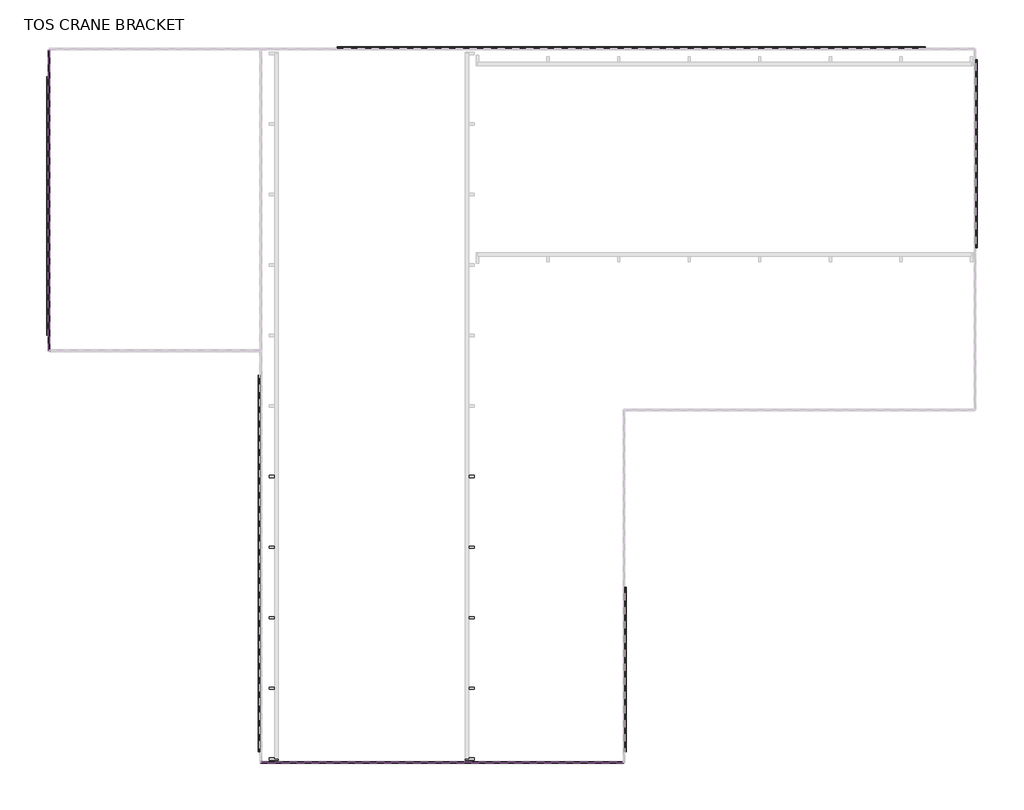
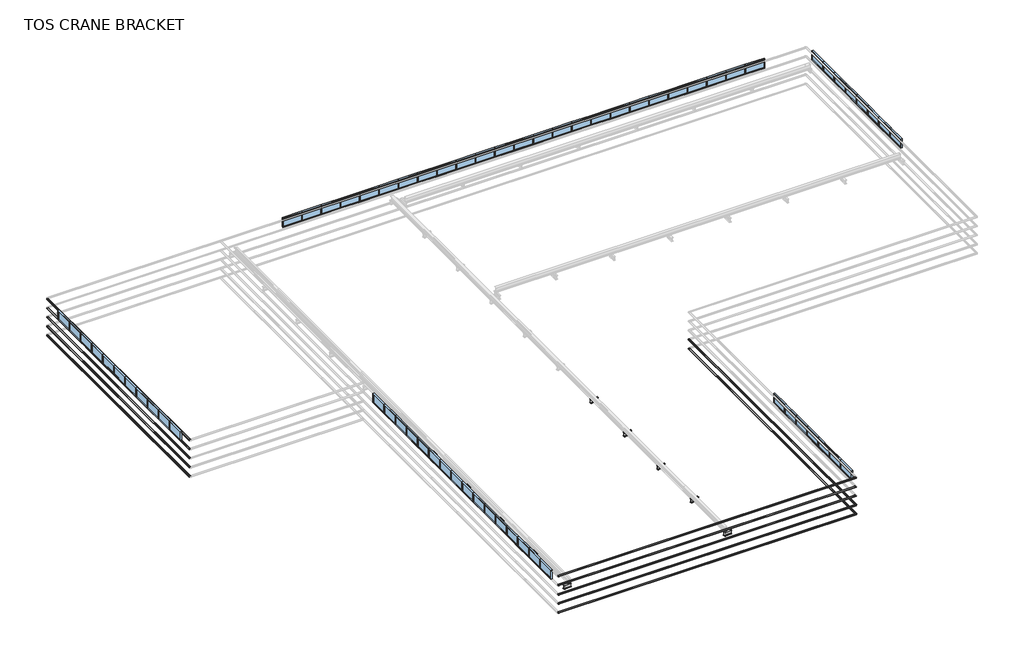
# One storey, part 1 of 3: 67 windows, 22 beams.
"""IFC4 building model written with IfcOpenShell, lengths in millimetres."""

import ifcopenshell
import ifcopenshell.guid

model = None  # the IFC model being written
_history = None  # IfcOwnerHistory: only IFC2X3 demands one
_inside = {}  # id of a spatial element -> (the spatial element, [elements in it])
_under = {}  # id of a project, library or spatial element -> (it, [spatial elements below it])
_declared = {}  # id of a project -> (the project, [libraries it declares])
_typed = {}  # id of a type object -> (the type object, [elements of that type])
_made_of = {}  # id of a material, layer set ... -> (it, [elements and type objects made of it])


def new_model(schema):
    """Start an empty IFC model of exactly this schema.

    Asked for "IFC4X3", IfcOpenShell would pick the latest addendum, in which some entities
    have other attributes; the version numbers below select the first issue.
    IFC2X3 requires an IfcOwnerHistory on every rooted entity: one is made here for all.
    """
    global model, _history
    if schema == "IFC4X3":
        model = ifcopenshell.file(schema_version=(4, 3, 0, 0))
    else:
        model = ifcopenshell.file(schema=schema)
    _inside.clear()
    _under.clear()
    _declared.clear()
    _typed.clear()
    _made_of.clear()
    _history = None
    if model.schema == "IFC2X3":
        org = make("IfcOrganization", Name="unknown")
        user = make(
            "IfcPersonAndOrganization",
            ThePerson=make("IfcPerson", FamilyName="unknown"),
            TheOrganization=org,
        )
        app = make(
            "IfcApplication",
            ApplicationDeveloper=org,
            Version="unknown",
            ApplicationFullName="unknown",
            ApplicationIdentifier="unknown",
        )
        _history = make(
            "IfcOwnerHistory",
            OwningUser=user,
            OwningApplication=app,
            ChangeAction="ADDED",
            CreationDate=0,
        )
    return model


def make(cls, **values):
    """One entity of the class cls with the attributes given. An attribute that is None is left unset."""
    return model.create_entity(
        cls, **{name: value for name, value in values.items() if value is not None}
    )


def rooted(cls, **values):
    """An entity with a GlobalId (a new one), such as an element, a storey or a relation."""
    return make(cls, GlobalId=ifcopenshell.guid.new(), OwnerHistory=_history, **values)


def si_unit(unit_type, name, prefix=None):
    """IfcSIUnit, for example si_unit("LENGTHUNIT", "METRE", prefix="MILLI")."""
    return make("IfcSIUnit", UnitType=unit_type, Prefix=prefix, Name=name)


def assignment(units):
    """IfcUnitAssignment: the units of a project."""
    return None if units is None else make("IfcUnitAssignment", Units=units)


def point(xyz):
    """IfcCartesianPoint."""
    return None if xyz is None else make("IfcCartesianPoint", Coordinates=xyz)


def direction(xyz):
    """IfcDirection."""
    return None if xyz is None else make("IfcDirection", DirectionRatios=xyz)


def frame(location, z_axis=None, x_axis=None):
    """IfcAxis2Placement3D, a coordinate frame: its origin and axes. An axis left out is left unset."""
    return make(
        "IfcAxis2Placement3D",
        Location=point(location),
        Axis=direction(z_axis),
        RefDirection=direction(x_axis),
    )


def frame_2d(location, x_axis=None):
    """IfcAxis2Placement2D, a coordinate frame in the plane: its origin and x axis."""
    return make(
        "IfcAxis2Placement2D", Location=point(location), RefDirection=direction(x_axis)
    )


def origin():
    """The frame at (0, 0, 0) with its axes left unset."""
    return frame((0.0, 0.0, 0.0))


def place(relative_to, where):
    """IfcLocalPlacement: puts the frame where relative to a parent placement (None: the world)."""
    return make(
        "IfcLocalPlacement", PlacementRelTo=relative_to, RelativePlacement=where
    )


def context(
    kind, dimensions, precision=None, world=None, true_north=None, identifier=None
):
    """IfcGeometricRepresentationContext, for example the 3D "Model" context."""
    return make(
        "IfcGeometricRepresentationContext",
        ContextIdentifier=identifier,
        ContextType=kind,
        CoordinateSpaceDimension=dimensions,
        Precision=precision,
        WorldCoordinateSystem=world,
        TrueNorth=true_north,
    )


def project(units=None, contexts=None):
    """IfcProject with its units and contexts."""
    return rooted(
        "IfcProject",
        Name="project",
        RepresentationContexts=contexts,
        UnitsInContext=assignment(units),
    )


def spatial(cls, under=None, at=None, **own):
    """A site, building, storey or space (cls), placed at a placement, below another one or the project."""
    s = rooted(cls, ObjectPlacement=at, **own)
    if under is not None:
        _under.setdefault(under.id(), (under, []))[1].append(s)
    return s


def polyline(points):
    """IfcPolyline through the points."""
    return make("IfcPolyline", Points=[point(p) for p in points])


def circle_curve(where, radius):
    """IfcCircle in the frame where."""
    return make("IfcCircle", Position=where, Radius=radius)


def trimmed(basis, trim1, trim2, sense, master):
    """IfcTrimmedCurve: the piece of a basis curve between two trims."""
    return make(
        "IfcTrimmedCurve",
        BasisCurve=basis,
        Trim1=trim1,
        Trim2=trim2,
        SenseAgreement=sense,
        MasterRepresentation=master,
    )


def segment(curve, same_sense, transition):
    """IfcCompositeCurveSegment."""
    return make(
        "IfcCompositeCurveSegment",
        Transition=transition,
        SameSense=same_sense,
        ParentCurve=curve,
    )


def composite_curve(segments, self_intersect=None):
    """IfcCompositeCurve: segments joined end to end."""
    return make("IfcCompositeCurve", Segments=segments, SelfIntersect=self_intersect)


def outline(outer, holes=None, kind="AREA"):
    """IfcArbitraryClosedProfileDef: a profile drawn as a closed curve; with holes, ...WithVoids."""
    if holes is None:
        return make("IfcArbitraryClosedProfileDef", ProfileType=kind, OuterCurve=outer)
    return make(
        "IfcArbitraryProfileDefWithVoids",
        ProfileType=kind,
        OuterCurve=outer,
        InnerCurves=holes,
    )


def extrude(swept, where, along, depth):
    """IfcExtrudedAreaSolid: the profile swept, set in the frame where, extruded along a direction by depth."""
    return make(
        "IfcExtrudedAreaSolid",
        SweptArea=swept,
        Position=where,
        ExtrudedDirection=direction(along),
        Depth=depth,
    )


def shape(context_of_items, identifier, shape_type, items):
    """IfcShapeRepresentation: the items that make up one representation, for example the "Body"."""
    return make(
        "IfcShapeRepresentation",
        ContextOfItems=context_of_items,
        RepresentationIdentifier=identifier,
        RepresentationType=shape_type,
        Items=items,
    )


def source(mapping_origin, context_of_items, identifier, shape_type, items):
    """IfcRepresentationMap: a shape defined once, which mapped items show again and again."""
    return make(
        "IfcRepresentationMap",
        MappingOrigin=mapping_origin,
        MappedRepresentation=shape(context_of_items, identifier, shape_type, items),
    )


def transform(
    local_origin,
    x_axis=None,
    y_axis=None,
    z_axis=None,
    scale=None,
    scale2=None,
    scale3=None,
    uniform=True,
):
    """IfcCartesianTransformationOperator3D, or its non-uniform kind. x_axis, y_axis, z_axis: its Axis1, 2, 3."""
    if uniform:
        return make(
            "IfcCartesianTransformationOperator3D",
            Axis1=direction(x_axis),
            Axis2=direction(y_axis),
            LocalOrigin=point(local_origin),
            Scale=scale,
            Axis3=direction(z_axis),
        )
    return make(
        "IfcCartesianTransformationOperator3DnonUniform",
        Axis1=direction(x_axis),
        Axis2=direction(y_axis),
        LocalOrigin=point(local_origin),
        Scale=scale,
        Axis3=direction(z_axis),
        Scale2=scale2,
        Scale3=scale3,
    )


def mapped(mapping_source, mapping_target):
    """IfcMappedItem: shows the shape of a source again, moved by a transform."""
    return make(
        "IfcMappedItem", MappingSource=mapping_source, MappingTarget=mapping_target
    )


def made_of(thing, what):
    """Note that an element or type object is made of a material, layer set ...; save() writes the relation."""
    if what is not None:
        _made_of.setdefault(what.id(), (what, []))[1].append(thing)
    return thing


def element(
    cls,
    number,
    at=None,
    inside=None,
    cuts=None,
    type_object=None,
    material=None,
    context=None,
    identifier="Body",
    shape_type=None,
    held_by="IfcProductDefinitionShape",
    body=None,
    shapes=None,
    **own,
):
    """One element of the class cls, such as IfcWall. Its Tag is "e" and its number.

    at: its placement. inside: the storey or other place that contains it. cuts: it is an
    opening in that element (IfcRelVoidsElement). A single representation is given by context,
    identifier, shape_type and body (its items); several are given by shapes. held_by: the class
    of the entity that holds the representations. save() writes the other relations.
    """
    e = rooted(cls, Tag="e%d" % number, ObjectPlacement=at, **own)
    if body is not None:
        shapes = [shape(context, identifier, shape_type, body)]
    if shapes is not None:
        e.Representation = make(held_by, Representations=shapes)
    if inside is not None:
        _inside.setdefault(inside.id(), (inside, []))[1].append(e)
    if cuts is not None:
        rooted(
            "IfcRelVoidsElement", RelatingBuildingElement=cuts, RelatedOpeningElement=e
        )
    if type_object is not None:
        _typed.setdefault(type_object.id(), (type_object, []))[1].append(e)
    return made_of(e, material)


def aggregate(whole, parts):
    """IfcRelAggregates: a whole, such as a stair, and the parts it consists of."""
    return rooted("IfcRelAggregates", RelatingObject=whole, RelatedObjects=parts)


def save(model, path):
    """Write the relations noted so far, then the file.

    IfcRelAggregates (storeys below a building ...), IfcRelContainedInSpatialStructure (elements
    in a storey), IfcRelDefinesByType, IfcRelAssociatesMaterial and IfcRelDeclares: one each for
    every whole, place, type object, material and project.
    """
    for whole, parts in _under.values():
        aggregate(whole, parts)
    for where, things in _inside.values():
        rooted(
            "IfcRelContainedInSpatialStructure",
            RelatedElements=things,
            RelatingStructure=where,
        )
    for kind, things in _typed.values():
        rooted("IfcRelDefinesByType", RelatedObjects=things, RelatingType=kind)
    for what, things in _made_of.values():
        rooted("IfcRelAssociatesMaterial", RelatedObjects=things, RelatingMaterial=what)
    for by, libraries in _declared.values():
        rooted("IfcRelDeclares", RelatingContext=by, RelatedDefinitions=libraries)
    model.write(path)


def beam_a081c7c9(model_context):
    return source(origin(), model_context, "Body", "SweptSolid", [
        extrude(outline(composite_curve([segment(polyline([(100.0, -187.0), (100.0, -200.0), (-100.0, -200.0), (-100.0, -187.0), (-20.0, -187.0)]), True, "CONTINUOUS"), segment(trimmed(circle_curve(frame_2d((-20.0, -171.0)), 16.0), [point((-20.0, -187.0))], [point((-4.0, -171.0))], True, "CARTESIAN"), True, "CONTINUOUS"), segment(polyline([(-4.0, -171.0), (-4.0, 171.0)]), True, "CONTINUOUS"), segment(trimmed(circle_curve(frame_2d((-20.0, 171.0)), 16.0), [point((-4.0, 171.0))], [point((-20.0, 187.0))], True, "CARTESIAN"), True, "CONTINUOUS"), segment(polyline([(-20.0, 187.0), (-100.0, 187.0), (-100.0, 200.0), (100.0, 200.0), (100.0, 187.0), (20.0, 187.0)]), True, "CONTINUOUS"), segment(trimmed(circle_curve(frame_2d((20.0, 171.0)), 16.0), [point((20.0, 187.0))], [point((4.0, 171.0))], True, "CARTESIAN"), True, "CONTINUOUS"), segment(polyline([(4.0, 171.0), (4.0, -171.0)]), True, "CONTINUOUS"), segment(trimmed(circle_curve(frame_2d((20.0, -171.0)), 16.0), [point((4.0, -171.0))], [point((20.0, -187.0))], True, "CARTESIAN"), True, "CONTINUOUS"), segment(polyline([(20.0, -187.0), (100.0, -187.0)]), True, "CONTINUOUS")], self_intersect=False)), frame((-236.0, 0.0, 0.0), z_axis=(1.0, 0.0, 0.0), x_axis=(0.0, 1.0, 0.0)), (0.0, 0.0, 1.0), 766.0),
    ])


def beam_d36fe593(model_context):
    return source(origin(), model_context, "Body", "SweptSolid", [
        extrude(outline(composite_curve([segment(polyline([(-100.0, -187.0), (-20.0, -187.0)]), True, "CONTINUOUS"), segment(trimmed(circle_curve(frame_2d((-20.0, -171.0)), 16.0), [point((-20.0, -187.0))], [point((-4.0, -171.0))], True, "CARTESIAN"), True, "CONTINUOUS"), segment(polyline([(-4.0, -171.0), (-4.0, 171.0)]), True, "CONTINUOUS"), segment(trimmed(circle_curve(frame_2d((-20.0, 171.0)), 16.0), [point((-4.0, 171.0))], [point((-20.0, 187.0))], True, "CARTESIAN"), True, "CONTINUOUS"), segment(polyline([(-20.0, 187.0), (-100.0, 187.0), (-100.0, 200.0), (100.0, 200.0), (100.0, 187.0), (20.0, 187.0)]), True, "CONTINUOUS"), segment(trimmed(circle_curve(frame_2d((20.0, 171.0)), 16.0), [point((20.0, 187.0))], [point((4.0, 171.0))], True, "CARTESIAN"), True, "CONTINUOUS"), segment(polyline([(4.0, 171.0), (4.0, -171.0)]), True, "CONTINUOUS"), segment(trimmed(circle_curve(frame_2d((20.0, -171.0)), 16.0), [point((4.0, -171.0))], [point((20.0, -187.0))], True, "CARTESIAN"), True, "CONTINUOUS"), segment(polyline([(20.0, -187.0), (100.0, -187.0), (100.0, -200.0), (-100.0, -200.0), (-100.0, -187.0)]), True, "CONTINUOUS")], self_intersect=False)), frame((-236.0, 0.0, 0.0), z_axis=(1.0, 0.0, 0.0), x_axis=(0.0, 1.0, 0.0)), (0.0, 0.0, 1.0), 766.0),
    ])


def steel_framing_lc_f9ca99c4(model_context):
    return source(origin(), model_context, "Body", "SweptSolid", [
        extrude(outline(composite_curve([segment(polyline([(18.6, 67.0), (18.6, -67.0)]), True, "CONTINUOUS"), segment(trimmed(circle_curve(frame_2d((10.6, -67.0)), 8.0), [point((18.6, -67.0))], [point((10.6, -75.0))], False, "CARTESIAN"), True, "CONTINUOUS"), segment(polyline([(10.6, -75.0), (-48.4, -75.0)]), True, "CONTINUOUS"), segment(trimmed(circle_curve(frame_2d((-48.4, -67.0)), 8.0), [point((-48.4, -75.0))], [point((-56.4, -67.0))], False, "CARTESIAN"), True, "CONTINUOUS"), segment(polyline([(-56.4, -67.0), (-56.4, -50.0), (-53.2, -50.0), (-53.2, -67.0)]), True, "CONTINUOUS"), segment(trimmed(circle_curve(frame_2d((-48.4, -67.0)), 4.8), [point((-53.2, -67.0))], [point((-48.4, -71.8))], True, "CARTESIAN"), True, "CONTINUOUS"), segment(polyline([(-48.4, -71.8), (10.6, -71.8)]), True, "CONTINUOUS"), segment(trimmed(circle_curve(frame_2d((10.6, -67.0)), 4.8), [point((10.6, -71.8))], [point((15.4, -67.0))], True, "CARTESIAN"), True, "CONTINUOUS"), segment(polyline([(15.4, -67.0), (15.4, 67.0)]), True, "CONTINUOUS"), segment(trimmed(circle_curve(frame_2d((10.6, 67.0)), 4.8), [point((15.4, 67.0))], [point((10.6, 71.8))], True, "CARTESIAN"), True, "CONTINUOUS"), segment(polyline([(10.6, 71.8), (-48.4, 71.8)]), True, "CONTINUOUS"), segment(trimmed(circle_curve(frame_2d((-48.4, 67.0)), 4.8), [point((-48.4, 71.8))], [point((-53.2, 67.0))], True, "CARTESIAN"), True, "CONTINUOUS"), segment(polyline([(-53.2, 67.0), (-53.2, 50.0), (-56.4, 50.0), (-56.4, 67.0)]), True, "CONTINUOUS"), segment(trimmed(circle_curve(frame_2d((-48.4, 67.0)), 8.0), [point((-56.4, 67.0))], [point((-48.4, 75.0))], False, "CARTESIAN"), True, "CONTINUOUS"), segment(polyline([(-48.4, 75.0), (10.6, 75.0)]), True, "CONTINUOUS"), segment(trimmed(circle_curve(frame_2d((10.6, 67.0)), 8.0), [point((10.6, 75.0))], [point((18.6, 67.0))], False, "CARTESIAN"), True, "CONTINUOUS")], self_intersect=False)), frame((-12797.0, 0.0, 0.0), z_axis=(1.0, 0.0, 0.0), x_axis=(0.0, 1.0, 0.0)), (0.0, 0.0, 1.0), 25581.0),
    ])


def steel_framing_lc_7a68255c(model_context):
    return source(origin(), model_context, "Body", "SweptSolid", [
        extrude(outline(composite_curve([segment(polyline([(18.6, 67.0), (18.6, -67.0)]), True, "CONTINUOUS"), segment(trimmed(circle_curve(frame_2d((10.6, -67.0)), 8.0), [point((18.6, -67.0))], [point((10.6, -75.0))], False, "CARTESIAN"), True, "CONTINUOUS"), segment(polyline([(10.6, -75.0), (-48.4, -75.0)]), True, "CONTINUOUS"), segment(trimmed(circle_curve(frame_2d((-48.4, -67.0)), 8.0), [point((-48.4, -75.0))], [point((-56.4, -67.0))], False, "CARTESIAN"), True, "CONTINUOUS"), segment(polyline([(-56.4, -67.0), (-56.4, -50.0), (-53.2, -50.0), (-53.2, -67.0)]), True, "CONTINUOUS"), segment(trimmed(circle_curve(frame_2d((-48.4, -67.0)), 4.8), [point((-53.2, -67.0))], [point((-48.4, -71.8))], True, "CARTESIAN"), True, "CONTINUOUS"), segment(polyline([(-48.4, -71.8), (10.6, -71.8)]), True, "CONTINUOUS"), segment(trimmed(circle_curve(frame_2d((10.6, -67.0)), 4.8), [point((10.6, -71.8))], [point((15.4, -67.0))], True, "CARTESIAN"), True, "CONTINUOUS"), segment(polyline([(15.4, -67.0), (15.4, 67.0)]), True, "CONTINUOUS"), segment(trimmed(circle_curve(frame_2d((10.6, 67.0)), 4.8), [point((15.4, 67.0))], [point((10.6, 71.8))], True, "CARTESIAN"), True, "CONTINUOUS"), segment(polyline([(10.6, 71.8), (-48.4, 71.8)]), True, "CONTINUOUS"), segment(trimmed(circle_curve(frame_2d((-48.4, 67.0)), 4.8), [point((-48.4, 71.8))], [point((-53.2, 67.0))], True, "CARTESIAN"), True, "CONTINUOUS"), segment(polyline([(-53.2, 67.0), (-53.2, 50.0), (-56.4, 50.0), (-56.4, 67.0)]), True, "CONTINUOUS"), segment(trimmed(circle_curve(frame_2d((-48.4, 67.0)), 8.0), [point((-56.4, 67.0))], [point((-48.4, 75.0))], False, "CARTESIAN"), True, "CONTINUOUS"), segment(polyline([(-48.4, 75.0), (10.6, 75.0)]), True, "CONTINUOUS"), segment(trimmed(circle_curve(frame_2d((10.6, 67.0)), 8.0), [point((10.6, 75.0))], [point((18.6, 67.0))], False, "CARTESIAN"), True, "CONTINUOUS")], self_intersect=False)), frame((-15450.0, 0.0, 0.0), z_axis=(1.0, 0.0, 0.0), x_axis=(0.0, 1.0, 0.0)), (0.0, 0.0, 1.0), 30900.0),
    ])


def fixed_window_a76b3388(model_context):
    return source(origin(), model_context, "Body", "SweptSolid", [
        extrude(outline(polyline([(-950.0, 3.0), (950.0, 3.0), (950.0, -3.0), (-950.0, -3.0), (-950.0, 3.0)])), frame((0.0, 0.0, 850.0), z_axis=(0.0, 0.0, 1.0), x_axis=(1.0, 0.0, 0.0)), (0.0, 0.0, 1.0), 900.0),
        extrude(outline(polyline([(1800.0, -1000.0), (800.0, -1000.0), (800.0, 1000.0), (1800.0, 1000.0), (1800.0, -1000.0)]), holes=[polyline([(1750.0, -950.0), (1750.0, 950.0), (850.0, 950.0), (850.0, -950.0), (1750.0, -950.0)])]), frame((0.0, -75.0, 0.0), z_axis=(0.0, 1.0, 0.0), x_axis=(0.0, 0.0, 1.0)), (0.0, 0.0, 1.0), 150.0),
    ])


model = new_model("IFC4")

# Units and contexts
model_context = context("Model", 3, world=origin())
ifc_project = project(units=[si_unit("LENGTHUNIT", "METRE", prefix="MILLI")], contexts=[model_context])

# Site, building, storey
site = spatial("IfcSite", under=ifc_project)
building = spatial("IfcBuilding", under=site)
storey = spatial("IfcBuildingStorey", under=building, Name="TOS CRANE BRACKET", Elevation=6699.9618634)

# Beams
placement = place(None, origin())
beam_shape = beam_a081c7c9(model_context)
element("IfcBeam", 1, ObjectType="Steel Framing_H_KS : H_SB_AR_S02_H-400x200x8x13_SCB1", at=placement, inside=storey, context=model_context, shape_type="MappedRepresentation", body=[
    mapped(beam_shape, transform((35470.0, -36000.0, 6499.9618634), x_axis=(-1.0, 0.0, 0.0), y_axis=(0.0, -1.0, 0.0), z_axis=(0.0, 0.0, 1.0))),
])
element("IfcBeam", 2, ObjectType="Steel Framing_H_KS : H_SB_AR_S02_H-400x200x8x13_SCB1", at=placement, inside=storey, context=model_context, shape_type="MappedRepresentation", body=[
    mapped(beam_shape, transform((35470.0, -42000.0, 6499.9618634), x_axis=(-1.0, 0.0, 0.0), y_axis=(0.0, -1.0, 0.0), z_axis=(0.0, 0.0, 1.0))),
])
element("IfcBeam", 3, ObjectType="Steel Framing_H_KS : H_SB_AR_S02_H-400x200x8x13_SCB1", at=placement, inside=storey, context=model_context, shape_type="MappedRepresentation", body=[
    mapped(beam_shape, transform((35470.0, -48000.0, 6499.9618634), x_axis=(-1.0, 0.0, 0.0), y_axis=(0.0, -1.0, 0.0), z_axis=(0.0, 0.0, 1.0))),
])
element("IfcBeam", 4, ObjectType="Steel Framing_H_KS : H_SB_AR_S02_H-400x200x8x13_SCB1", at=placement, inside=storey, context=model_context, shape_type="MappedRepresentation", body=[
    mapped(beam_shape, transform((35470.0, -54000.0, 6499.9618634), x_axis=(-1.0, 0.0, 0.0), y_axis=(0.0, -1.0, 0.0), z_axis=(0.0, 0.0, 1.0))),
])
element("IfcBeam", 5, ObjectType="Steel Framing_H_KS : H_SB_AR_S02_H-400x200x8x13_SCB1", at=placement, inside=storey, context=model_context, shape_type="MappedRepresentation", body=[
    mapped(beam_shape, transform((35470.0, -60000.0, 6499.9618634), x_axis=(-1.0, 0.0, 0.0), y_axis=(0.0, -1.0, 0.0), z_axis=(0.0, 0.0, 1.0))),
])
beam_2_shape = beam_d36fe593(model_context)
element("IfcBeam", 6, ObjectType="Steel Framing_H_KS : H_SB_AR_S02_H-400x200x8x13_SCB1", at=placement, inside=storey, context=model_context, shape_type="MappedRepresentation", body=[
    mapped(beam_2_shape, transform((18530.0, -36000.0, 6499.9618634), x_axis=(1.0, 0.0, 0.0), y_axis=(0.0, 1.0, 0.0), z_axis=(0.0, 0.0, 1.0))),
])
element("IfcBeam", 7, ObjectType="Steel Framing_H_KS : H_SB_AR_S02_H-400x200x8x13_SCB1", at=placement, inside=storey, context=model_context, shape_type="MappedRepresentation", body=[
    mapped(beam_2_shape, transform((18530.0, -42000.0, 6499.9618634), x_axis=(1.0, 0.0, 0.0), y_axis=(0.0, 1.0, 0.0), z_axis=(0.0, 0.0, 1.0))),
])
element("IfcBeam", 8, ObjectType="Steel Framing_H_KS : H_SB_AR_S02_H-400x200x8x13_SCB1", at=placement, inside=storey, context=model_context, shape_type="MappedRepresentation", body=[
    mapped(beam_2_shape, transform((18530.0, -48000.0, 6499.9618634), x_axis=(1.0, 0.0, 0.0), y_axis=(0.0, 1.0, 0.0), z_axis=(0.0, 0.0, 1.0))),
])
element("IfcBeam", 9, ObjectType="Steel Framing_H_KS : H_SB_AR_S02_H-400x200x8x13_SCB1", at=placement, inside=storey, context=model_context, shape_type="MappedRepresentation", body=[
    mapped(beam_2_shape, transform((18530.0, -54000.0, 6499.9618634), x_axis=(1.0, 0.0, 0.0), y_axis=(0.0, 1.0, 0.0), z_axis=(0.0, 0.0, 1.0))),
])
element("IfcBeam", 10, ObjectType="Steel Framing_H_KS : H_SB_AR_S02_H-400x200x8x13_SCB1", at=placement, inside=storey, context=model_context, shape_type="MappedRepresentation", body=[
    mapped(beam_2_shape, transform((18530.0, -60000.0, 6499.9618634), x_axis=(1.0, 0.0, 0.0), y_axis=(0.0, 1.0, 0.0), z_axis=(0.0, 0.0, 1.0))),
])
element("IfcBeam", 11, ObjectType="Steel Framing_LC : H_SB_AR_S00_LC-150x75x25x3.2", at=placement, inside=storey, context=model_context, shape_type="SweptSolid", body=[
    extrude(outline(composite_curve([segment(polyline([(4168.5618634, 48517.0), (4168.5618634, 48383.0)]), True, "CONTINUOUS"), segment(trimmed(circle_curve(frame_2d((4160.5618634, 48383.0)), 8.0), [point((4168.5618634, 48383.0))], [point((4160.5618634, 48375.0))], False, "CARTESIAN"), True, "CONTINUOUS"), segment(polyline([(4160.5618634, 48375.0), (4101.5618634, 48375.0)]), True, "CONTINUOUS"), segment(trimmed(circle_curve(frame_2d((4101.5618634, 48383.0)), 8.0), [point((4101.5618634, 48375.0))], [point((4093.5618634, 48383.0))], False, "CARTESIAN"), True, "CONTINUOUS"), segment(polyline([(4093.5618634, 48383.0), (4093.5618634, 48400.0), (4096.7618634, 48400.0), (4096.7618634, 48383.0)]), True, "CONTINUOUS"), segment(trimmed(circle_curve(frame_2d((4101.5618634, 48383.0)), 4.8), [point((4096.7618634, 48383.0))], [point((4101.5618634, 48378.2))], True, "CARTESIAN"), True, "CONTINUOUS"), segment(polyline([(4101.5618634, 48378.2), (4160.5618634, 48378.2)]), True, "CONTINUOUS"), segment(trimmed(circle_curve(frame_2d((4160.5618634, 48383.0)), 4.8), [point((4160.5618634, 48378.2))], [point((4165.3618634, 48383.0))], True, "CARTESIAN"), True, "CONTINUOUS"), segment(polyline([(4165.3618634, 48383.0), (4165.3618634, 48517.0)]), True, "CONTINUOUS"), segment(trimmed(circle_curve(frame_2d((4160.5618634, 48517.0)), 4.8), [point((4165.3618634, 48517.0))], [point((4160.5618634, 48521.8))], True, "CARTESIAN"), True, "CONTINUOUS"), segment(polyline([(4160.5618634, 48521.8), (4101.5618634, 48521.8)]), True, "CONTINUOUS"), segment(trimmed(circle_curve(frame_2d((4101.5618634, 48517.0)), 4.8), [point((4101.5618634, 48521.8))], [point((4096.7618634, 48517.0))], True, "CARTESIAN"), True, "CONTINUOUS"), segment(polyline([(4096.7618634, 48517.0), (4096.7618634, 48500.0), (4093.5618634, 48500.0), (4093.5618634, 48517.0)]), True, "CONTINUOUS"), segment(trimmed(circle_curve(frame_2d((4101.5618634, 48517.0)), 8.0), [point((4093.5618634, 48517.0))], [point((4101.5618634, 48525.0))], False, "CARTESIAN"), True, "CONTINUOUS"), segment(polyline([(4101.5618634, 48525.0), (4160.5618634, 48525.0)]), True, "CONTINUOUS"), segment(trimmed(circle_curve(frame_2d((4160.5618634, 48517.0)), 8.0), [point((4160.5618634, 48525.0))], [point((4168.5618634, 48517.0))], False, "CARTESIAN"), True, "CONTINUOUS")], self_intersect=False)), frame((0.0, -60300.0, 0.0), z_axis=(0.0, 1.0, 0.0), x_axis=(0.0, 0.0, 1.0)), (0.0, 0.0, 1.0), 29975.0),
])
element("IfcBeam", 12, ObjectType="Steel Framing_LC : H_SB_AR_S00_LC-150x75x25x3.2", at=placement, inside=storey, context=model_context, shape_type="SweptSolid", body=[
    extrude(outline(composite_curve([segment(polyline([(5168.5618634, 48517.0), (5168.5618634, 48383.0)]), True, "CONTINUOUS"), segment(trimmed(circle_curve(frame_2d((5160.5618634, 48383.0)), 8.0), [point((5168.5618634, 48383.0))], [point((5160.5618634, 48375.0))], False, "CARTESIAN"), True, "CONTINUOUS"), segment(polyline([(5160.5618634, 48375.0), (5101.5618634, 48375.0)]), True, "CONTINUOUS"), segment(trimmed(circle_curve(frame_2d((5101.5618634, 48383.0)), 8.0), [point((5101.5618634, 48375.0))], [point((5093.5618634, 48383.0))], False, "CARTESIAN"), True, "CONTINUOUS"), segment(polyline([(5093.5618634, 48383.0), (5093.5618634, 48400.0), (5096.7618634, 48400.0), (5096.7618634, 48383.0)]), True, "CONTINUOUS"), segment(trimmed(circle_curve(frame_2d((5101.5618634, 48383.0)), 4.8), [point((5096.7618634, 48383.0))], [point((5101.5618634, 48378.2))], True, "CARTESIAN"), True, "CONTINUOUS"), segment(polyline([(5101.5618634, 48378.2), (5160.5618634, 48378.2)]), True, "CONTINUOUS"), segment(trimmed(circle_curve(frame_2d((5160.5618634, 48383.0)), 4.8), [point((5160.5618634, 48378.2))], [point((5165.3618634, 48383.0))], True, "CARTESIAN"), True, "CONTINUOUS"), segment(polyline([(5165.3618634, 48383.0), (5165.3618634, 48517.0)]), True, "CONTINUOUS"), segment(trimmed(circle_curve(frame_2d((5160.5618634, 48517.0)), 4.8), [point((5165.3618634, 48517.0))], [point((5160.5618634, 48521.8))], True, "CARTESIAN"), True, "CONTINUOUS"), segment(polyline([(5160.5618634, 48521.8), (5101.5618634, 48521.8)]), True, "CONTINUOUS"), segment(trimmed(circle_curve(frame_2d((5101.5618634, 48517.0)), 4.8), [point((5101.5618634, 48521.8))], [point((5096.7618634, 48517.0))], True, "CARTESIAN"), True, "CONTINUOUS"), segment(polyline([(5096.7618634, 48517.0), (5096.7618634, 48500.0), (5093.5618634, 48500.0), (5093.5618634, 48517.0)]), True, "CONTINUOUS"), segment(trimmed(circle_curve(frame_2d((5101.5618634, 48517.0)), 8.0), [point((5093.5618634, 48517.0))], [point((5101.5618634, 48525.0))], False, "CARTESIAN"), True, "CONTINUOUS"), segment(polyline([(5101.5618634, 48525.0), (5160.5618634, 48525.0)]), True, "CONTINUOUS"), segment(trimmed(circle_curve(frame_2d((5160.5618634, 48517.0)), 8.0), [point((5160.5618634, 48525.0))], [point((5168.5618634, 48517.0))], False, "CARTESIAN"), True, "CONTINUOUS")], self_intersect=False)), frame((0.0, -60300.0, 0.0), z_axis=(0.0, 1.0, 0.0), x_axis=(0.0, 0.0, 1.0)), (0.0, 0.0, 1.0), 29975.0),
])
steel_framing_lc_shape = steel_framing_lc_f9ca99c4(model_context)
element("IfcBeam", 13, ObjectType="Steel Framing_LC : H_SB_AR_S00_LC-150x75x25x3.2", at=placement, inside=storey, context=model_context, shape_type="MappedRepresentation", body=[
    mapped(steel_framing_lc_shape, transform((-450.0, -12503.0, 4149.9618634), x_axis=(0.0, 1.0, 0.0), y_axis=(0.0, 0.0, 1.0), z_axis=(1.0, 0.0, 0.0))),
])
element("IfcBeam", 14, ObjectType="Steel Framing_LC : H_SB_AR_S00_LC-150x75x25x3.2", at=placement, inside=storey, context=model_context, shape_type="MappedRepresentation", body=[
    mapped(steel_framing_lc_shape, transform((-450.0, -12503.0, 5149.9618634), x_axis=(0.0, 1.0, 0.0), y_axis=(0.0, 0.0, 1.0), z_axis=(1.0, 0.0, 0.0))),
])
element("IfcBeam", 15, ObjectType="Steel Framing_LC : H_SB_AR_S00_LC-150x75x25x3.2", at=placement, inside=storey, context=model_context, shape_type="MappedRepresentation", body=[
    mapped(steel_framing_lc_shape, transform((-450.0, -12503.0, 6149.9618634), x_axis=(0.0, 1.0, 0.0), y_axis=(0.0, 0.0, 1.0), z_axis=(1.0, 0.0, 0.0))),
])
element("IfcBeam", 16, ObjectType="Steel Framing_LC : H_SB_AR_S00_LC-150x75x25x3.2", at=placement, inside=storey, context=model_context, shape_type="MappedRepresentation", body=[
    mapped(steel_framing_lc_shape, transform((-450.0, -12503.0, 7149.9618634), x_axis=(0.0, 1.0, 0.0), y_axis=(0.0, 0.0, 1.0), z_axis=(1.0, 0.0, 0.0))),
])
element("IfcBeam", 17, ObjectType="Steel Framing_LC : H_SB_AR_S00_LC-150x75x25x3.2", at=placement, inside=storey, context=model_context, shape_type="MappedRepresentation", body=[
    mapped(steel_framing_lc_shape, transform((-450.0, -12503.0, 8149.9618634), x_axis=(0.0, 1.0, 0.0), y_axis=(0.0, 0.0, 1.0), z_axis=(1.0, 0.0, 0.0))),
])
steel_framing_lc_2_shape = steel_framing_lc_7a68255c(model_context)
element("IfcBeam", 18, ObjectType="Steel Framing_LC : H_SB_AR_S00_LC-150x75x25x3.2", at=placement, inside=storey, context=model_context, shape_type="MappedRepresentation", body=[
    mapped(steel_framing_lc_2_shape, transform((33000.0, -60300.0, 4149.9618634), x_axis=(1.0, 0.0, 0.0), y_axis=(0.0, 0.0, 1.0), z_axis=(0.0, -1.0, 0.0))),
])
element("IfcBeam", 19, ObjectType="Steel Framing_LC : H_SB_AR_S00_LC-150x75x25x3.2", at=placement, inside=storey, context=model_context, shape_type="MappedRepresentation", body=[
    mapped(steel_framing_lc_2_shape, transform((33000.0, -60300.0, 5149.9618634), x_axis=(1.0, 0.0, 0.0), y_axis=(0.0, 0.0, 1.0), z_axis=(0.0, -1.0, 0.0))),
])
element("IfcBeam", 20, ObjectType="Steel Framing_LC : H_SB_AR_S00_LC-150x75x25x3.2", at=placement, inside=storey, context=model_context, shape_type="MappedRepresentation", body=[
    mapped(steel_framing_lc_2_shape, transform((33000.0, -60300.0, 6149.9618634), x_axis=(1.0, 0.0, 0.0), y_axis=(0.0, 0.0, 1.0), z_axis=(0.0, -1.0, 0.0))),
])
element("IfcBeam", 21, ObjectType="Steel Framing_LC : H_SB_AR_S00_LC-150x75x25x3.2", at=placement, inside=storey, context=model_context, shape_type="MappedRepresentation", body=[
    mapped(steel_framing_lc_2_shape, transform((33000.0, -60300.0, 7149.9618634), x_axis=(1.0, 0.0, 0.0), y_axis=(0.0, 0.0, 1.0), z_axis=(0.0, -1.0, 0.0))),
])
element("IfcBeam", 22, ObjectType="Steel Framing_LC : H_SB_AR_S00_LC-150x75x25x3.2", at=placement, inside=storey, context=model_context, shape_type="MappedRepresentation", body=[
    mapped(steel_framing_lc_2_shape, transform((33000.0, -60300.0, 8149.9618634), x_axis=(1.0, 0.0, 0.0), y_axis=(0.0, 0.0, 1.0), z_axis=(0.0, -1.0, 0.0))),
])

# Windows
fixed_window_shape = fixed_window_a76b3388(model_context)
element("IfcWindow", 23, ObjectType="Fixed Window : H_WD_AR_B11_Fix_Steel Window_SG_W2000xH1000", at=placement, inside=storey, context=model_context, shape_type="MappedRepresentation", body=[
    mapped(fixed_window_shape, transform((-585.0, -22975.0, 6499.9618634), x_axis=(0.0, 1.0, 0.0), y_axis=(-1.0, 0.0, 0.0), z_axis=(0.0, 0.0, 1.0))),
])
element("IfcWindow", 24, ObjectType="Fixed Window : H_WD_AR_B11_Fix_Steel Window_SG_W2000xH1000", at=placement, inside=storey, context=model_context, shape_type="MappedRepresentation", body=[
    mapped(fixed_window_shape, transform((-585.0, -20975.0, 6499.9618634), x_axis=(0.0, -1.0, 0.0), y_axis=(1.0, 0.0, 0.0), z_axis=(0.0, 0.0, 1.0))),
])
element("IfcWindow", 25, ObjectType="Fixed Window : H_WD_AR_B11_Fix_Steel Window_SG_W2000xH1000", at=placement, inside=storey, context=model_context, shape_type="MappedRepresentation", body=[
    mapped(fixed_window_shape, transform((-585.0, -18975.0, 6499.9618634), x_axis=(0.0, -1.0, 0.0), y_axis=(1.0, 0.0, 0.0), z_axis=(0.0, 0.0, 1.0))),
])
element("IfcWindow", 26, ObjectType="Fixed Window : H_WD_AR_B11_Fix_Steel Window_SG_W2000xH1000", at=placement, inside=storey, context=model_context, shape_type="MappedRepresentation", body=[
    mapped(fixed_window_shape, transform((-585.0, -16975.0, 6499.9618634), x_axis=(0.0, -1.0, 0.0), y_axis=(1.0, 0.0, 0.0), z_axis=(0.0, 0.0, 1.0))),
])
element("IfcWindow", 27, ObjectType="Fixed Window : H_WD_AR_B11_Fix_Steel Window_SG_W2000xH1000", at=placement, inside=storey, context=model_context, shape_type="MappedRepresentation", body=[
    mapped(fixed_window_shape, transform((-585.0, -14975.0, 6499.9618634), x_axis=(0.0, -1.0, 0.0), y_axis=(1.0, 0.0, 0.0), z_axis=(0.0, 0.0, 1.0))),
])
element("IfcWindow", 28, ObjectType="Fixed Window : H_WD_AR_B11_Fix_Steel Window_SG_W2000xH1000", at=placement, inside=storey, context=model_context, shape_type="MappedRepresentation", body=[
    mapped(fixed_window_shape, transform((-585.0, -12975.0, 6499.9618634), x_axis=(0.0, -1.0, 0.0), y_axis=(1.0, 0.0, 0.0), z_axis=(0.0, 0.0, 1.0))),
])
element("IfcWindow", 29, ObjectType="Fixed Window : H_WD_AR_B11_Fix_Steel Window_SG_W2000xH1000", at=placement, inside=storey, context=model_context, shape_type="MappedRepresentation", body=[
    mapped(fixed_window_shape, transform((-585.0, -10975.0, 6499.9618634), x_axis=(0.0, -1.0, 0.0), y_axis=(1.0, 0.0, 0.0), z_axis=(0.0, 0.0, 1.0))),
])
element("IfcWindow", 30, ObjectType="Fixed Window : H_WD_AR_B11_Fix_Steel Window_SG_W2000xH1000", at=placement, inside=storey, context=model_context, shape_type="MappedRepresentation", body=[
    mapped(fixed_window_shape, transform((-585.0, -8975.0, 6499.9618634), x_axis=(0.0, -1.0, 0.0), y_axis=(1.0, 0.0, 0.0), z_axis=(0.0, 0.0, 1.0))),
])
element("IfcWindow", 31, ObjectType="Fixed Window : H_WD_AR_B11_Fix_Steel Window_SG_W2000xH1000", at=placement, inside=storey, context=model_context, shape_type="MappedRepresentation", body=[
    mapped(fixed_window_shape, transform((-585.0, -6975.0, 6499.9618634), x_axis=(0.0, -1.0, 0.0), y_axis=(1.0, 0.0, 0.0), z_axis=(0.0, 0.0, 1.0))),
])
element("IfcWindow", 32, ObjectType="Fixed Window : H_WD_AR_B11_Fix_Steel Window_SG_W2000xH1000", at=placement, inside=storey, context=model_context, shape_type="MappedRepresentation", body=[
    mapped(fixed_window_shape, transform((-585.0, -4975.0, 6499.9618634), x_axis=(0.0, -1.0, 0.0), y_axis=(1.0, 0.0, 0.0), z_axis=(0.0, 0.0, 1.0))),
])
element("IfcWindow", 33, ObjectType="Fixed Window : H_WD_AR_B11_Fix_Steel Window_SG_W2000xH1000", at=placement, inside=storey, context=model_context, shape_type="MappedRepresentation", body=[
    mapped(fixed_window_shape, transform((-585.0, -2975.0, 6499.9618634), x_axis=(0.0, -1.0, 0.0), y_axis=(1.0, 0.0, 0.0), z_axis=(0.0, 0.0, 1.0))),
])
element("IfcWindow", 34, ObjectType="Fixed Window : H_WD_AR_B11_Fix_Steel Window_SG_W2000xH1000", at=placement, inside=storey, context=model_context, shape_type="MappedRepresentation", body=[
    mapped(fixed_window_shape, transform((25075.0, 504.0, 6499.9618634), x_axis=(1.0, 0.0, 0.0), y_axis=(0.0, 1.0, 0.0), z_axis=(0.0, 0.0, 1.0))),
])
element("IfcWindow", 35, ObjectType="Fixed Window : H_WD_AR_B11_Fix_Steel Window_SG_W2000xH1000", at=placement, inside=storey, context=model_context, shape_type="MappedRepresentation", body=[
    mapped(fixed_window_shape, transform((27075.0, 504.0, 6499.9618634), x_axis=(1.0, 0.0, 0.0), y_axis=(0.0, 1.0, 0.0), z_axis=(0.0, 0.0, 1.0))),
])
element("IfcWindow", 36, ObjectType="Fixed Window : H_WD_AR_B11_Fix_Steel Window_SG_W2000xH1000", at=placement, inside=storey, context=model_context, shape_type="MappedRepresentation", body=[
    mapped(fixed_window_shape, transform((29075.0, 504.0, 6499.9618634), x_axis=(1.0, 0.0, 0.0), y_axis=(0.0, 1.0, 0.0), z_axis=(0.0, 0.0, 1.0))),
])
element("IfcWindow", 37, ObjectType="Fixed Window : H_WD_AR_B11_Fix_Steel Window_SG_W2000xH1000", at=placement, inside=storey, context=model_context, shape_type="MappedRepresentation", body=[
    mapped(fixed_window_shape, transform((31075.0, 504.0, 6499.9618634), x_axis=(-1.0, 0.0, 0.0), y_axis=(0.0, -1.0, 0.0), z_axis=(0.0, 0.0, 1.0))),
])
element("IfcWindow", 38, ObjectType="Fixed Window : H_WD_AR_B11_Fix_Steel Window_SG_W2000xH1000", at=placement, inside=storey, context=model_context, shape_type="MappedRepresentation", body=[
    mapped(fixed_window_shape, transform((33075.0, 504.0, 6499.9618634), x_axis=(1.0, 0.0, 0.0), y_axis=(0.0, 1.0, 0.0), z_axis=(0.0, 0.0, 1.0))),
])
element("IfcWindow", 39, ObjectType="Fixed Window : H_WD_AR_B11_Fix_Steel Window_SG_W2000xH1000", at=placement, inside=storey, context=model_context, shape_type="MappedRepresentation", body=[
    mapped(fixed_window_shape, transform((35075.0, 504.0, 6499.9618634), x_axis=(1.0, 0.0, 0.0), y_axis=(0.0, 1.0, 0.0), z_axis=(0.0, 0.0, 1.0))),
])
element("IfcWindow", 40, ObjectType="Fixed Window : H_WD_AR_B11_Fix_Steel Window_SG_W2000xH1000", at=placement, inside=storey, context=model_context, shape_type="MappedRepresentation", body=[
    mapped(fixed_window_shape, transform((37075.0, 504.0, 6499.9618634), x_axis=(1.0, 0.0, 0.0), y_axis=(0.0, 1.0, 0.0), z_axis=(0.0, 0.0, 1.0))),
])
element("IfcWindow", 41, ObjectType="Fixed Window : H_WD_AR_B11_Fix_Steel Window_SG_W2000xH1000", at=placement, inside=storey, context=model_context, shape_type="MappedRepresentation", body=[
    mapped(fixed_window_shape, transform((39075.0, 504.0, 6499.9618634), x_axis=(1.0, 0.0, 0.0), y_axis=(0.0, 1.0, 0.0), z_axis=(0.0, 0.0, 1.0))),
])
element("IfcWindow", 42, ObjectType="Fixed Window : H_WD_AR_B11_Fix_Steel Window_SG_W2000xH1000", at=placement, inside=storey, context=model_context, shape_type="MappedRepresentation", body=[
    mapped(fixed_window_shape, transform((41075.0, 504.0, 6499.9618634), x_axis=(1.0, 0.0, 0.0), y_axis=(0.0, 1.0, 0.0), z_axis=(0.0, 0.0, 1.0))),
])
element("IfcWindow", 43, ObjectType="Fixed Window : H_WD_AR_B11_Fix_Steel Window_SG_W2000xH1000", at=placement, inside=storey, context=model_context, shape_type="MappedRepresentation", body=[
    mapped(fixed_window_shape, transform((43075.0, 504.0, 6499.9618634), x_axis=(-1.0, 0.0, 0.0), y_axis=(0.0, -1.0, 0.0), z_axis=(0.0, 0.0, 1.0))),
])
element("IfcWindow", 44, ObjectType="Fixed Window : H_WD_AR_B11_Fix_Steel Window_SG_W2000xH1000", at=placement, inside=storey, context=model_context, shape_type="MappedRepresentation", body=[
    mapped(fixed_window_shape, transform((45075.0, 504.0, 6499.9618634), x_axis=(1.0, 0.0, 0.0), y_axis=(0.0, 1.0, 0.0), z_axis=(0.0, 0.0, 1.0))),
])
element("IfcWindow", 45, ObjectType="Fixed Window : H_WD_AR_B11_Fix_Steel Window_SG_W2000xH1000", at=placement, inside=storey, context=model_context, shape_type="MappedRepresentation", body=[
    mapped(fixed_window_shape, transform((47075.0, 504.0, 6499.9618634), x_axis=(1.0, 0.0, 0.0), y_axis=(0.0, 1.0, 0.0), z_axis=(0.0, 0.0, 1.0))),
])
element("IfcWindow", 46, ObjectType="Fixed Window : H_WD_AR_B11_Fix_Steel Window_SG_W2000xH1000", at=placement, inside=storey, context=model_context, shape_type="MappedRepresentation", body=[
    mapped(fixed_window_shape, transform((49075.0, 504.0, 6499.9618634), x_axis=(1.0, 0.0, 0.0), y_axis=(0.0, 1.0, 0.0), z_axis=(0.0, 0.0, 1.0))),
])
element("IfcWindow", 47, ObjectType="Fixed Window : H_WD_AR_B11_Fix_Steel Window_SG_W2000xH1000", at=placement, inside=storey, context=model_context, shape_type="MappedRepresentation", body=[
    mapped(fixed_window_shape, transform((51075.0, 504.0, 6499.9618634), x_axis=(1.0, 0.0, 0.0), y_axis=(0.0, 1.0, 0.0), z_axis=(0.0, 0.0, 1.0))),
])
element("IfcWindow", 48, ObjectType="Fixed Window : H_WD_AR_B11_Fix_Steel Window_SG_W2000xH1000", at=placement, inside=storey, context=model_context, shape_type="MappedRepresentation", body=[
    mapped(fixed_window_shape, transform((53075.0, 504.0, 6499.9618634), x_axis=(1.0, 0.0, 0.0), y_axis=(0.0, 1.0, 0.0), z_axis=(0.0, 0.0, 1.0))),
])
element("IfcWindow", 49, ObjectType="Fixed Window : H_WD_AR_B11_Fix_Steel Window_SG_W2000xH1000", at=placement, inside=storey, context=model_context, shape_type="MappedRepresentation", body=[
    mapped(fixed_window_shape, transform((55075.0, 504.0, 6499.9618634), x_axis=(1.0, 0.0, 0.0), y_axis=(0.0, 1.0, 0.0), z_axis=(0.0, 0.0, 1.0))),
])
element("IfcWindow", 50, ObjectType="Fixed Window : H_WD_AR_B11_Fix_Steel Window_SG_W2000xH1000", at=placement, inside=storey, context=model_context, shape_type="MappedRepresentation", body=[
    mapped(fixed_window_shape, transform((57075.0, 504.0, 6499.9618634), x_axis=(1.0, 0.0, 0.0), y_axis=(0.0, 1.0, 0.0), z_axis=(0.0, 0.0, 1.0))),
])
element("IfcWindow", 51, ObjectType="Fixed Window : H_WD_AR_B11_Fix_Steel Window_SG_W2000xH1000", at=placement, inside=storey, context=model_context, shape_type="MappedRepresentation", body=[
    mapped(fixed_window_shape, transform((59075.0, 504.0, 6499.9618634), x_axis=(1.0, 0.0, 0.0), y_axis=(0.0, 1.0, 0.0), z_axis=(0.0, 0.0, 1.0))),
])
element("IfcWindow", 52, ObjectType="Fixed Window : H_WD_AR_B11_Fix_Steel Window_SG_W2000xH1000", at=placement, inside=storey, context=model_context, shape_type="MappedRepresentation", body=[
    mapped(fixed_window_shape, transform((61075.0, 504.0, 6499.9618634), x_axis=(1.0, 0.0, 0.0), y_axis=(0.0, 1.0, 0.0), z_axis=(0.0, 0.0, 1.0))),
])
element("IfcWindow", 53, ObjectType="Fixed Window : H_WD_AR_B11_Fix_Steel Window_SG_W2000xH1000", at=placement, inside=storey, context=model_context, shape_type="MappedRepresentation", body=[
    mapped(fixed_window_shape, transform((63075.0, 504.0, 6499.9618634), x_axis=(1.0, 0.0, 0.0), y_axis=(0.0, 1.0, 0.0), z_axis=(0.0, 0.0, 1.0))),
])
element("IfcWindow", 54, ObjectType="Fixed Window : H_WD_AR_B11_Fix_Steel Window_SG_W2000xH1000", at=placement, inside=storey, context=model_context, shape_type="MappedRepresentation", body=[
    mapped(fixed_window_shape, transform((65075.0, 504.0, 6499.9618634), x_axis=(1.0, 0.0, 0.0), y_axis=(0.0, 1.0, 0.0), z_axis=(0.0, 0.0, 1.0))),
])
element("IfcWindow", 55, ObjectType="Fixed Window : H_WD_AR_B11_Fix_Steel Window_SG_W2000xH1000", at=placement, inside=storey, context=model_context, shape_type="MappedRepresentation", body=[
    mapped(fixed_window_shape, transform((67075.0, 504.0, 6499.9618634), x_axis=(1.0, 0.0, 0.0), y_axis=(0.0, 1.0, 0.0), z_axis=(0.0, 0.0, 1.0))),
])
element("IfcWindow", 56, ObjectType="Fixed Window : H_WD_AR_B11_Fix_Steel Window_SG_W2000xH1000", at=placement, inside=storey, context=model_context, shape_type="MappedRepresentation", body=[
    mapped(fixed_window_shape, transform((69075.0, 504.0, 6499.9618634), x_axis=(1.0, 0.0, 0.0), y_axis=(0.0, 1.0, 0.0), z_axis=(0.0, 0.0, 1.0))),
])
element("IfcWindow", 57, ObjectType="Fixed Window : H_WD_AR_B11_Fix_Steel Window_SG_W2000xH1000", at=placement, inside=storey, context=model_context, shape_type="MappedRepresentation", body=[
    mapped(fixed_window_shape, transform((71075.0, 504.0, 6499.9618634), x_axis=(1.0, 0.0, 0.0), y_axis=(0.0, 1.0, 0.0), z_axis=(0.0, 0.0, 1.0))),
])
element("IfcWindow", 58, ObjectType="Fixed Window : H_WD_AR_B11_Fix_Steel Window_SG_W2000xH1000", at=placement, inside=storey, context=model_context, shape_type="MappedRepresentation", body=[
    mapped(fixed_window_shape, transform((73075.0, 504.0, 6499.9618634), x_axis=(1.0, 0.0, 0.0), y_axis=(0.0, 1.0, 0.0), z_axis=(0.0, 0.0, 1.0))),
])
element("IfcWindow", 59, ObjectType="Fixed Window : H_WD_AR_B11_Fix_Steel Window_SG_W2000xH1000", at=placement, inside=storey, context=model_context, shape_type="MappedRepresentation", body=[
    mapped(fixed_window_shape, transform((78435.0, -1556.0, 6499.9618634), x_axis=(0.0, -1.0, 0.0), y_axis=(1.0, 0.0, 0.0), z_axis=(0.0, 0.0, 1.0))),
])
element("IfcWindow", 60, ObjectType="Fixed Window : H_WD_AR_B11_Fix_Steel Window_SG_W2000xH1000", at=placement, inside=storey, context=model_context, shape_type="MappedRepresentation", body=[
    mapped(fixed_window_shape, transform((78435.0, -3556.0, 6499.9618634), x_axis=(0.0, -1.0, 0.0), y_axis=(1.0, 0.0, 0.0), z_axis=(0.0, 0.0, 1.0))),
])
element("IfcWindow", 61, ObjectType="Fixed Window : H_WD_AR_B11_Fix_Steel Window_SG_W2000xH1000", at=placement, inside=storey, context=model_context, shape_type="MappedRepresentation", body=[
    mapped(fixed_window_shape, transform((78435.0, -5556.0, 6499.9618634), x_axis=(0.0, -1.0, 0.0), y_axis=(1.0, 0.0, 0.0), z_axis=(0.0, 0.0, 1.0))),
])
element("IfcWindow", 62, ObjectType="Fixed Window : H_WD_AR_B11_Fix_Steel Window_SG_W2000xH1000", at=placement, inside=storey, context=model_context, shape_type="MappedRepresentation", body=[
    mapped(fixed_window_shape, transform((78435.0, -7556.0, 6499.9618634), x_axis=(0.0, -1.0, 0.0), y_axis=(1.0, 0.0, 0.0), z_axis=(0.0, 0.0, 1.0))),
])
element("IfcWindow", 63, ObjectType="Fixed Window : H_WD_AR_B11_Fix_Steel Window_SG_W2000xH1000", at=placement, inside=storey, context=model_context, shape_type="MappedRepresentation", body=[
    mapped(fixed_window_shape, transform((78435.0, -9556.0, 6499.9618634), x_axis=(0.0, -1.0, 0.0), y_axis=(1.0, 0.0, 0.0), z_axis=(0.0, 0.0, 1.0))),
])
element("IfcWindow", 64, ObjectType="Fixed Window : H_WD_AR_B11_Fix_Steel Window_SG_W2000xH1000", at=placement, inside=storey, context=model_context, shape_type="MappedRepresentation", body=[
    mapped(fixed_window_shape, transform((78435.0, -11556.0, 6499.9618634), x_axis=(0.0, -1.0, 0.0), y_axis=(1.0, 0.0, 0.0), z_axis=(0.0, 0.0, 1.0))),
])
element("IfcWindow", 65, ObjectType="Fixed Window : H_WD_AR_B11_Fix_Steel Window_SG_W2000xH1000", at=placement, inside=storey, context=model_context, shape_type="MappedRepresentation", body=[
    mapped(fixed_window_shape, transform((78435.0, -13556.0, 6499.9618634), x_axis=(0.0, -1.0, 0.0), y_axis=(1.0, 0.0, 0.0), z_axis=(0.0, 0.0, 1.0))),
])
element("IfcWindow", 66, ObjectType="Fixed Window : H_WD_AR_B11_Fix_Steel Window_SG_W2000xH1000", at=placement, inside=storey, context=model_context, shape_type="MappedRepresentation", body=[
    mapped(fixed_window_shape, transform((78435.0, -15550.0, 6499.9618634), x_axis=(0.0, 1.0, 0.0), y_axis=(-1.0, 0.0, 0.0), z_axis=(0.0, 0.0, 1.0))),
])
element("IfcWindow", 67, ObjectType="Fixed Window : H_WD_AR_B11_Fix_Steel Window_SG_W2000xH1000", at=placement, inside=storey, context=model_context, shape_type="MappedRepresentation", body=[
    mapped(fixed_window_shape, transform((48585.0, -58375.0, 6499.9618634), x_axis=(0.0, -1.0, 0.0), y_axis=(1.0, 0.0, 0.0), z_axis=(0.0, 0.0, 1.0))),
])
element("IfcWindow", 68, ObjectType="Fixed Window : H_WD_AR_B11_Fix_Steel Window_SG_W2000xH1000", at=placement, inside=storey, context=model_context, shape_type="MappedRepresentation", body=[
    mapped(fixed_window_shape, transform((48585.0, -56375.0, 6499.9618634), x_axis=(0.0, -1.0, 0.0), y_axis=(1.0, 0.0, 0.0), z_axis=(0.0, 0.0, 1.0))),
])
element("IfcWindow", 69, ObjectType="Fixed Window : H_WD_AR_B11_Fix_Steel Window_SG_W2000xH1000", at=placement, inside=storey, context=model_context, shape_type="MappedRepresentation", body=[
    mapped(fixed_window_shape, transform((48585.0, -54375.0, 6499.9618634), x_axis=(0.0, -1.0, 0.0), y_axis=(1.0, 0.0, 0.0), z_axis=(0.0, 0.0, 1.0))),
])
element("IfcWindow", 70, ObjectType="Fixed Window : H_WD_AR_B11_Fix_Steel Window_SG_W2000xH1000", at=placement, inside=storey, context=model_context, shape_type="MappedRepresentation", body=[
    mapped(fixed_window_shape, transform((48585.0, -52375.0, 6499.9618634), x_axis=(0.0, -1.0, 0.0), y_axis=(1.0, 0.0, 0.0), z_axis=(0.0, 0.0, 1.0))),
])
element("IfcWindow", 71, ObjectType="Fixed Window : H_WD_AR_B11_Fix_Steel Window_SG_W2000xH1000", at=placement, inside=storey, context=model_context, shape_type="MappedRepresentation", body=[
    mapped(fixed_window_shape, transform((48585.0, -50375.0, 6499.9618634), x_axis=(0.0, -1.0, 0.0), y_axis=(1.0, 0.0, 0.0), z_axis=(0.0, 0.0, 1.0))),
])
element("IfcWindow", 72, ObjectType="Fixed Window : H_WD_AR_B11_Fix_Steel Window_SG_W2000xH1000", at=placement, inside=storey, context=model_context, shape_type="MappedRepresentation", body=[
    mapped(fixed_window_shape, transform((48585.0, -48375.0, 6499.9618634), x_axis=(0.0, -1.0, 0.0), y_axis=(1.0, 0.0, 0.0), z_axis=(0.0, 0.0, 1.0))),
])
element("IfcWindow", 73, ObjectType="Fixed Window : H_WD_AR_B11_Fix_Steel Window_SG_W2000xH1000", at=placement, inside=storey, context=model_context, shape_type="MappedRepresentation", body=[
    mapped(fixed_window_shape, transform((48585.0, -46400.0, 6499.9618634), x_axis=(0.0, -1.0, 0.0), y_axis=(1.0, 0.0, 0.0), z_axis=(0.0, 0.0, 1.0))),
])
element("IfcWindow", 74, ObjectType="Fixed Window : H_WD_AR_B11_Fix_Steel Window_SG_W2000xH1000", at=placement, inside=storey, context=model_context, shape_type="MappedRepresentation", body=[
    mapped(fixed_window_shape, transform((17415.0, -58375.0, 6499.9618634), x_axis=(0.0, 1.0, 0.0), y_axis=(-1.0, 0.0, 0.0), z_axis=(0.0, 0.0, 1.0))),
])
element("IfcWindow", 75, ObjectType="Fixed Window : H_WD_AR_B11_Fix_Steel Window_SG_W2000xH1000", at=placement, inside=storey, context=model_context, shape_type="MappedRepresentation", body=[
    mapped(fixed_window_shape, transform((17415.0, -56375.0, 6499.9618634), x_axis=(0.0, 1.0, 0.0), y_axis=(-1.0, 0.0, 0.0), z_axis=(0.0, 0.0, 1.0))),
])
element("IfcWindow", 76, ObjectType="Fixed Window : H_WD_AR_B11_Fix_Steel Window_SG_W2000xH1000", at=placement, inside=storey, context=model_context, shape_type="MappedRepresentation", body=[
    mapped(fixed_window_shape, transform((17415.0, -54375.0, 6499.9618634), x_axis=(0.0, 1.0, 0.0), y_axis=(-1.0, 0.0, 0.0), z_axis=(0.0, 0.0, 1.0))),
])
element("IfcWindow", 77, ObjectType="Fixed Window : H_WD_AR_B11_Fix_Steel Window_SG_W2000xH1000", at=placement, inside=storey, context=model_context, shape_type="MappedRepresentation", body=[
    mapped(fixed_window_shape, transform((17415.0, -52375.0, 6499.9618634), x_axis=(0.0, -1.0, 0.0), y_axis=(1.0, 0.0, 0.0), z_axis=(0.0, 0.0, 1.0))),
])
element("IfcWindow", 78, ObjectType="Fixed Window : H_WD_AR_B11_Fix_Steel Window_SG_W2000xH1000", at=placement, inside=storey, context=model_context, shape_type="MappedRepresentation", body=[
    mapped(fixed_window_shape, transform((17415.0, -50375.0, 6499.9618634), x_axis=(0.0, 1.0, 0.0), y_axis=(-1.0, 0.0, 0.0), z_axis=(0.0, 0.0, 1.0))),
])
element("IfcWindow", 79, ObjectType="Fixed Window : H_WD_AR_B11_Fix_Steel Window_SG_W2000xH1000", at=placement, inside=storey, context=model_context, shape_type="MappedRepresentation", body=[
    mapped(fixed_window_shape, transform((17415.0, -48375.0, 6499.9618634), x_axis=(0.0, 1.0, 0.0), y_axis=(-1.0, 0.0, 0.0), z_axis=(0.0, 0.0, 1.0))),
])
element("IfcWindow", 80, ObjectType="Fixed Window : H_WD_AR_B11_Fix_Steel Window_SG_W2000xH1000", at=placement, inside=storey, context=model_context, shape_type="MappedRepresentation", body=[
    mapped(fixed_window_shape, transform((17415.0, -46375.0, 6499.9618634), x_axis=(0.0, -1.0, 0.0), y_axis=(1.0, 0.0, 0.0), z_axis=(0.0, 0.0, 1.0))),
])
element("IfcWindow", 81, ObjectType="Fixed Window : H_WD_AR_B11_Fix_Steel Window_SG_W2000xH1000", at=placement, inside=storey, context=model_context, shape_type="MappedRepresentation", body=[
    mapped(fixed_window_shape, transform((17415.0, -44375.0, 6499.9618634), x_axis=(0.0, -1.0, 0.0), y_axis=(1.0, 0.0, 0.0), z_axis=(0.0, 0.0, 1.0))),
])
element("IfcWindow", 82, ObjectType="Fixed Window : H_WD_AR_B11_Fix_Steel Window_SG_W2000xH1000", at=placement, inside=storey, context=model_context, shape_type="MappedRepresentation", body=[
    mapped(fixed_window_shape, transform((17415.0, -42375.0, 6499.9618634), x_axis=(0.0, 1.0, 0.0), y_axis=(-1.0, 0.0, 0.0), z_axis=(0.0, 0.0, 1.0))),
])
element("IfcWindow", 83, ObjectType="Fixed Window : H_WD_AR_B11_Fix_Steel Window_SG_W2000xH1000", at=placement, inside=storey, context=model_context, shape_type="MappedRepresentation", body=[
    mapped(fixed_window_shape, transform((17415.0, -40375.0, 6499.9618634), x_axis=(0.0, 1.0, 0.0), y_axis=(-1.0, 0.0, 0.0), z_axis=(0.0, 0.0, 1.0))),
])
element("IfcWindow", 84, ObjectType="Fixed Window : H_WD_AR_B11_Fix_Steel Window_SG_W2000xH1000", at=placement, inside=storey, context=model_context, shape_type="MappedRepresentation", body=[
    mapped(fixed_window_shape, transform((17415.0, -38375.0, 6499.9618634), x_axis=(0.0, -1.0, 0.0), y_axis=(1.0, 0.0, 0.0), z_axis=(0.0, 0.0, 1.0))),
])
element("IfcWindow", 85, ObjectType="Fixed Window : H_WD_AR_B11_Fix_Steel Window_SG_W2000xH1000", at=placement, inside=storey, context=model_context, shape_type="MappedRepresentation", body=[
    mapped(fixed_window_shape, transform((17415.0, -36375.0, 6499.9618634), x_axis=(0.0, -1.0, 0.0), y_axis=(1.0, 0.0, 0.0), z_axis=(0.0, 0.0, 1.0))),
])
element("IfcWindow", 86, ObjectType="Fixed Window : H_WD_AR_B11_Fix_Steel Window_SG_W2000xH1000", at=placement, inside=storey, context=model_context, shape_type="MappedRepresentation", body=[
    mapped(fixed_window_shape, transform((17415.0, -34375.0, 6499.9618634), x_axis=(0.0, -1.0, 0.0), y_axis=(1.0, 0.0, 0.0), z_axis=(0.0, 0.0, 1.0))),
])
element("IfcWindow", 87, ObjectType="Fixed Window : H_WD_AR_B11_Fix_Steel Window_SG_W2000xH1000", at=placement, inside=storey, context=model_context, shape_type="MappedRepresentation", body=[
    mapped(fixed_window_shape, transform((17415.0, -32375.0, 6499.9618634), x_axis=(0.0, -1.0, 0.0), y_axis=(1.0, 0.0, 0.0), z_axis=(0.0, 0.0, 1.0))),
])
element("IfcWindow", 88, ObjectType="Fixed Window : H_WD_AR_B11_Fix_Steel Window_SG_W2000xH1000", at=placement, inside=storey, context=model_context, shape_type="MappedRepresentation", body=[
    mapped(fixed_window_shape, transform((17415.0, -30375.0, 6499.9618634), x_axis=(0.0, 1.0, 0.0), y_axis=(-1.0, 0.0, 0.0), z_axis=(0.0, 0.0, 1.0))),
])
element("IfcWindow", 89, ObjectType="Fixed Window : H_WD_AR_B11_Fix_Steel Window_SG_W2000xH1000", at=placement, inside=storey, context=model_context, shape_type="MappedRepresentation", body=[
    mapped(fixed_window_shape, transform((17415.0, -28375.0, 6499.9618634), x_axis=(0.0, -1.0, 0.0), y_axis=(1.0, 0.0, 0.0), z_axis=(0.0, 0.0, 1.0))),
])

save(model, "model.ifc")

# Revit data of these elements
# Project information
#   H_Building Area = "0.00 m²"
#   H_Building H = "0"
#   H_Building L = "0"
#   H_Building NOS = "1"
#   H_Building Story = "1"
#   H_Building Total Area = "0.00 m²"
#   H_Building W = "0"
#   H_Building Volume = "0.000 m³"
#   H_Seismic Condition = "A as per ASCE 7-10"
#   H_Soil Condition = "C as per ASCE 7-10"
#   H_Basic Wind Speed = "58.3m/s ASCE7-10"
#   H_DS Project Code = "FAASA2302"
#   H_Project Abbreviation = "SACE2"
#   H_Project Division = "화공"
#   H_Project Finish = "2027-03-05"
#   H_Project Location = "Jafurah, Saudi Arabia"
#   H_Project Start = "2024-01-03"
#   H_Project Type = "EPC"
#   H_Smart Code = "FAASA2302"
#   Workset = "Project Info"
#   Project Issue Date = "Issue Date"
#   Project Status = "Project Status"
#   Client Name = "Owner"
#   Project Address = "Enter address here"
#   Project Name = "Project Name"
#   Project Number = "0001"
# Grids (mm)
#   "B": line (-13391.6, -6000) -> (80462.842, -6000)
#   "1": line (0, 6541.717) -> (0, -29558.74)
#   "2": line (6000, 6541.717) -> (6000, -29558.74)
#   "A": line (-13391.6, 0) -> (80462.842, 0)
#   "C": line (-13391.6, -12000) -> (80462.842, -12000)
#   "E-1": line (-13391.6, -25000) -> (19956.059, -25000)
#   "3": line (12000, 6541.717) -> (12000, -29558.74)
#   "4": line (18000, 6541.717) -> (18000, -63262.522)
#   "E": line (-13391.6, -24000) -> (80462.842, -24000)
#   "F": line (-13391.6, -30000) -> (80462.842, -30000)
#   "G": line (-13391.6, -36000) -> (49655.237, -36000)
#   "5": line (24000, 6541.717) -> (24000, -63262.522)
#   "6": line (30000, 6541.717) -> (30000, -63262.522)
#   "7": line (36000, 6541.717) -> (36000, -63262.522)
#   "8": line (42000, 6541.717) -> (42000, -63262.522)
#   "9": line (48000, 6541.717) -> (48000, -63262.522)
#   "10": line (54000, 6541.717) -> (54000, -33057.804)
#   "11": line (60000, 6541.717) -> (60000, -33057.804)
#   "12": line (66000, 6541.717) -> (66000, -33057.804)
#   "13": line (72000, 6541.717) -> (72000, -33057.804)
#   "14": line (78000, 6541.717) -> (78000, -33057.804)
#   "H": line (-13391.6, -42000) -> (49655.237, -42000)
#   "I": line (-13391.6, -48000) -> (49655.237, -48000)
